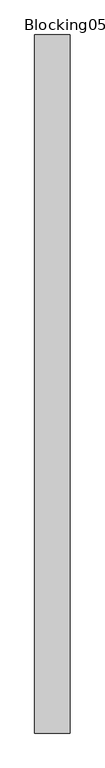
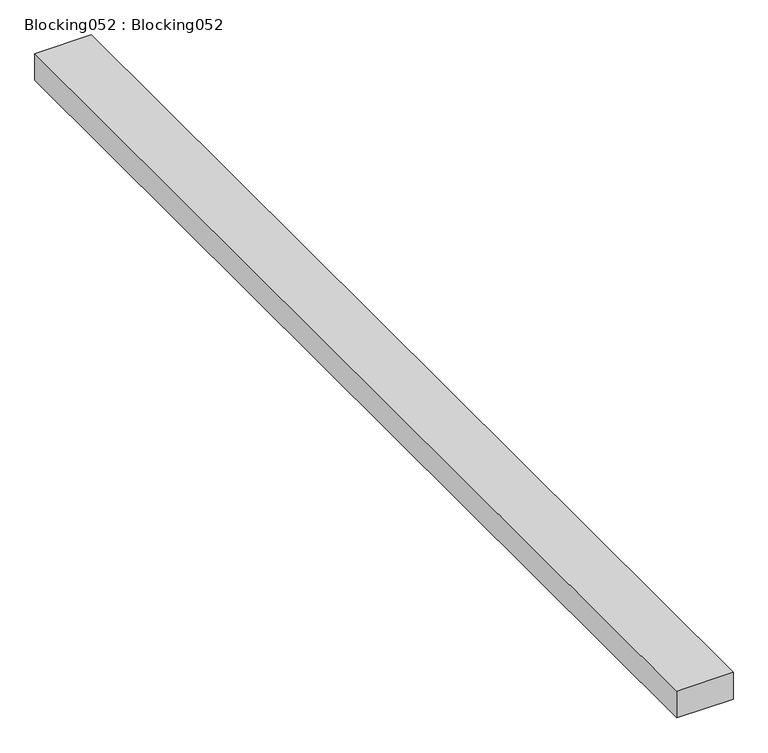
"""IFC4 building model written with IfcOpenShell, lengths in millimetres: proxy geometry, Blocking052 : Blocking052."""

import ifcopenshell
import ifcopenshell.guid

model = None  # the IFC model being written
_history = None  # IfcOwnerHistory: only IFC2X3 demands one
_inside = {}  # id of a spatial element -> (the spatial element, [elements in it])
_under = {}  # id of a project, library or spatial element -> (it, [spatial elements below it])
_declared = {}  # id of a project -> (the project, [libraries it declares])
_typed = {}  # id of a type object -> (the type object, [elements of that type])
_made_of = {}  # id of a material, layer set ... -> (it, [elements and type objects made of it])


def new_model(schema):
    """Start an empty IFC model of exactly this schema.

    Asked for "IFC4X3", IfcOpenShell would pick the latest addendum, in which some entities
    have other attributes; the version numbers below select the first issue.
    IFC2X3 requires an IfcOwnerHistory on every rooted entity: one is made here for all.
    """
    global model, _history
    if schema == "IFC4X3":
        model = ifcopenshell.file(schema_version=(4, 3, 0, 0))
    else:
        model = ifcopenshell.file(schema=schema)
    _inside.clear()
    _under.clear()
    _declared.clear()
    _typed.clear()
    _made_of.clear()
    _history = None
    if model.schema == "IFC2X3":
        org = make("IfcOrganization", Name="unknown")
        user = make(
            "IfcPersonAndOrganization",
            ThePerson=make("IfcPerson", FamilyName="unknown"),
            TheOrganization=org,
        )
        app = make(
            "IfcApplication",
            ApplicationDeveloper=org,
            Version="unknown",
            ApplicationFullName="unknown",
            ApplicationIdentifier="unknown",
        )
        _history = make(
            "IfcOwnerHistory",
            OwningUser=user,
            OwningApplication=app,
            ChangeAction="ADDED",
            CreationDate=0,
        )
    return model


def make(cls, **values):
    """One entity of the class cls with the attributes given. An attribute that is None is left unset."""
    return model.create_entity(
        cls, **{name: value for name, value in values.items() if value is not None}
    )


def rooted(cls, **values):
    """An entity with a GlobalId (a new one), such as an element, a storey or a relation."""
    return make(cls, GlobalId=ifcopenshell.guid.new(), OwnerHistory=_history, **values)


def si_unit(unit_type, name, prefix=None):
    """IfcSIUnit, for example si_unit("LENGTHUNIT", "METRE", prefix="MILLI")."""
    return make("IfcSIUnit", UnitType=unit_type, Prefix=prefix, Name=name)


def assignment(units):
    """IfcUnitAssignment: the units of a project."""
    return None if units is None else make("IfcUnitAssignment", Units=units)


def point(xyz):
    """IfcCartesianPoint."""
    return None if xyz is None else make("IfcCartesianPoint", Coordinates=xyz)


def direction(xyz):
    """IfcDirection."""
    return None if xyz is None else make("IfcDirection", DirectionRatios=xyz)


def frame(location, z_axis=None, x_axis=None):
    """IfcAxis2Placement3D, a coordinate frame: its origin and axes. An axis left out is left unset."""
    return make(
        "IfcAxis2Placement3D",
        Location=point(location),
        Axis=direction(z_axis),
        RefDirection=direction(x_axis),
    )


def origin():
    """The frame at (0, 0, 0) with its axes left unset."""
    return frame((0.0, 0.0, 0.0))


def place(relative_to, where):
    """IfcLocalPlacement: puts the frame where relative to a parent placement (None: the world)."""
    return make(
        "IfcLocalPlacement", PlacementRelTo=relative_to, RelativePlacement=where
    )


def context(
    kind, dimensions, precision=None, world=None, true_north=None, identifier=None
):
    """IfcGeometricRepresentationContext, for example the 3D "Model" context."""
    return make(
        "IfcGeometricRepresentationContext",
        ContextIdentifier=identifier,
        ContextType=kind,
        CoordinateSpaceDimension=dimensions,
        Precision=precision,
        WorldCoordinateSystem=world,
        TrueNorth=true_north,
    )


def project(units=None, contexts=None):
    """IfcProject with its units and contexts."""
    return rooted(
        "IfcProject",
        Name="project",
        RepresentationContexts=contexts,
        UnitsInContext=assignment(units),
    )


def spatial(cls, under=None, at=None, **own):
    """A site, building, storey or space (cls), placed at a placement, below another one or the project."""
    s = rooted(cls, ObjectPlacement=at, **own)
    if under is not None:
        _under.setdefault(under.id(), (under, []))[1].append(s)
    return s


def polyline(points):
    """IfcPolyline through the points."""
    return make("IfcPolyline", Points=[point(p) for p in points])


def outline(outer, holes=None, kind="AREA"):
    """IfcArbitraryClosedProfileDef: a profile drawn as a closed curve; with holes, ...WithVoids."""
    if holes is None:
        return make("IfcArbitraryClosedProfileDef", ProfileType=kind, OuterCurve=outer)
    return make(
        "IfcArbitraryProfileDefWithVoids",
        ProfileType=kind,
        OuterCurve=outer,
        InnerCurves=holes,
    )


def extrude(swept, where, along, depth):
    """IfcExtrudedAreaSolid: the profile swept, set in the frame where, extruded along a direction by depth."""
    return make(
        "IfcExtrudedAreaSolid",
        SweptArea=swept,
        Position=where,
        ExtrudedDirection=direction(along),
        Depth=depth,
    )


def shape(context_of_items, identifier, shape_type, items):
    """IfcShapeRepresentation: the items that make up one representation, for example the "Body"."""
    return make(
        "IfcShapeRepresentation",
        ContextOfItems=context_of_items,
        RepresentationIdentifier=identifier,
        RepresentationType=shape_type,
        Items=items,
    )


def source(mapping_origin, context_of_items, identifier, shape_type, items):
    """IfcRepresentationMap: a shape defined once, which mapped items show again and again."""
    return make(
        "IfcRepresentationMap",
        MappingOrigin=mapping_origin,
        MappedRepresentation=shape(context_of_items, identifier, shape_type, items),
    )


def transform(
    local_origin,
    x_axis=None,
    y_axis=None,
    z_axis=None,
    scale=None,
    scale2=None,
    scale3=None,
    uniform=True,
):
    """IfcCartesianTransformationOperator3D, or its non-uniform kind. x_axis, y_axis, z_axis: its Axis1, 2, 3."""
    if uniform:
        return make(
            "IfcCartesianTransformationOperator3D",
            Axis1=direction(x_axis),
            Axis2=direction(y_axis),
            LocalOrigin=point(local_origin),
            Scale=scale,
            Axis3=direction(z_axis),
        )
    return make(
        "IfcCartesianTransformationOperator3DnonUniform",
        Axis1=direction(x_axis),
        Axis2=direction(y_axis),
        LocalOrigin=point(local_origin),
        Scale=scale,
        Axis3=direction(z_axis),
        Scale2=scale2,
        Scale3=scale3,
    )


def mapped(mapping_source, mapping_target):
    """IfcMappedItem: shows the shape of a source again, moved by a transform."""
    return make(
        "IfcMappedItem", MappingSource=mapping_source, MappingTarget=mapping_target
    )


def made_of(thing, what):
    """Note that an element or type object is made of a material, layer set ...; save() writes the relation."""
    if what is not None:
        _made_of.setdefault(what.id(), (what, []))[1].append(thing)
    return thing


def element(
    cls,
    number,
    at=None,
    inside=None,
    cuts=None,
    type_object=None,
    material=None,
    context=None,
    identifier="Body",
    shape_type=None,
    held_by="IfcProductDefinitionShape",
    body=None,
    shapes=None,
    **own,
):
    """One element of the class cls, such as IfcWall. Its Tag is "e" and its number.

    at: its placement. inside: the storey or other place that contains it. cuts: it is an
    opening in that element (IfcRelVoidsElement). A single representation is given by context,
    identifier, shape_type and body (its items); several are given by shapes. held_by: the class
    of the entity that holds the representations. save() writes the other relations.
    """
    e = rooted(cls, Tag="e%d" % number, ObjectPlacement=at, **own)
    if body is not None:
        shapes = [shape(context, identifier, shape_type, body)]
    if shapes is not None:
        e.Representation = make(held_by, Representations=shapes)
    if inside is not None:
        _inside.setdefault(inside.id(), (inside, []))[1].append(e)
    if cuts is not None:
        rooted(
            "IfcRelVoidsElement", RelatingBuildingElement=cuts, RelatedOpeningElement=e
        )
    if type_object is not None:
        _typed.setdefault(type_object.id(), (type_object, []))[1].append(e)
    return made_of(e, material)


def aggregate(whole, parts):
    """IfcRelAggregates: a whole, such as a stair, and the parts it consists of."""
    return rooted("IfcRelAggregates", RelatingObject=whole, RelatedObjects=parts)


def save(model, path):
    """Write the relations noted so far, then the file.

    IfcRelAggregates (storeys below a building ...), IfcRelContainedInSpatialStructure (elements
    in a storey), IfcRelDefinesByType, IfcRelAssociatesMaterial and IfcRelDeclares: one each for
    every whole, place, type object, material and project.
    """
    for whole, parts in _under.values():
        aggregate(whole, parts)
    for where, things in _inside.values():
        rooted(
            "IfcRelContainedInSpatialStructure",
            RelatedElements=things,
            RelatingStructure=where,
        )
    for kind, things in _typed.values():
        rooted("IfcRelDefinesByType", RelatedObjects=things, RelatingType=kind)
    for what, things in _made_of.values():
        rooted("IfcRelAssociatesMaterial", RelatedObjects=things, RelatingMaterial=what)
    for by, libraries in _declared.values():
        rooted("IfcRelDeclares", RelatingContext=by, RelatedDefinitions=libraries)
    model.write(path)


def blocking052_blocking052_5466fccd(model_context):
    return source(origin(), model_context, "Body", "SweptSolid", [
        extrude(outline(polyline([(-9787.3237014, 7982.1531721), (-9888.9237014, 7982.1531721), (-9888.9237014, 9982.1531721), (-9787.3237014, 9982.1531721), (-9787.3237014, 7982.1531721)])), frame((0.0, 0.0, 40004.7460083), z_axis=(0.0, 0.0, 1.0), x_axis=(1.0, 0.0, 0.0)), (0.0, 0.0, 1.0), 50.8),
    ])


if __name__ == "__main__":
    model = new_model("IFC4")
    model_context = context("Model", 3, world=origin())
    ifc_project = project(units=[si_unit("LENGTHUNIT", "METRE", prefix="MILLI")], contexts=[model_context])
    site = spatial("IfcSite", under=ifc_project)
    building = spatial("IfcBuilding", under=site)
    placement = place(None, origin())
    blocking052_blocking052_shape = blocking052_blocking052_5466fccd(model_context)
    element("IfcBuildingElementProxy", 1, Name="Blocking052 : Blocking052", ObjectType="Blocking052 : Blocking052", at=placement, inside=building, context=model_context, shape_type="MappedRepresentation", body=[
        mapped(blocking052_blocking052_shape, transform((0.0, 0.0, 0.0), x_axis=(1.0, 0.0, 0.0), y_axis=(0.0, 1.0, 0.0), z_axis=(0.0, 0.0, 1.0))),
    ])
    save(model, "model.ifc")

# Revit data of these elements
# Type "Blocking052 : Blocking052"
#   NameOverride = "Blocking052"
# Element 1 (IfcBuildingElementProxy, "Blocking052 : Blocking052")
#   Materials on its faces: "WOOD BLOCKING AS REQUIRED"
# Materials
#   "WOOD BLOCKING AS REQUIRED": class "Unassigned", colour RGB 166 124 85, transparency 0, Cost = 0
